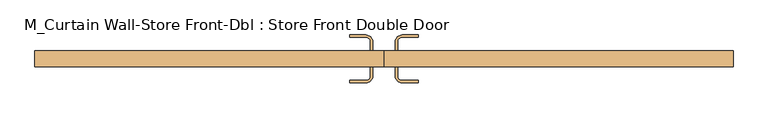
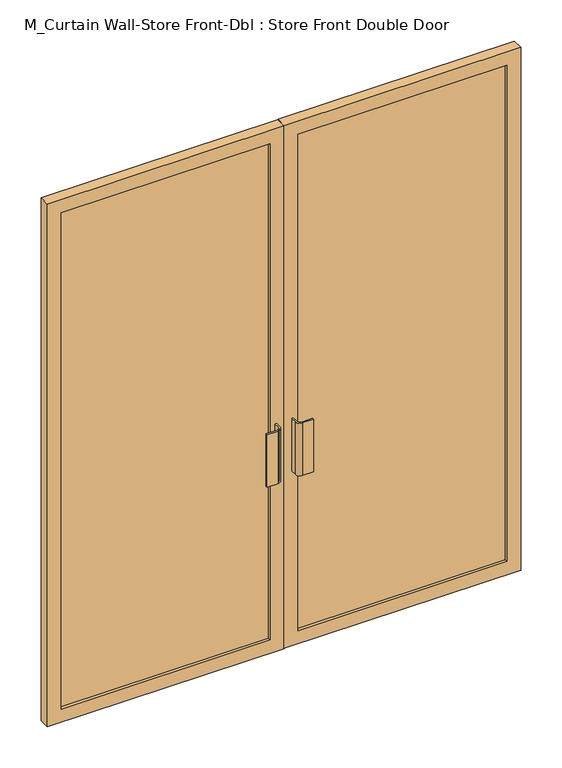
"""IFC4 building model written with IfcOpenShell, lengths in millimetres: door geometry, M_Curtain Wall-Store Front-Dbl : Store Front Double Door."""

from ifc_helpers import new_model, si_unit, point, frame, frame_2d, origin, place, context, project, spatial, polyline, circle_curve, trimmed, segment, composite_curve, outline, extrude, source, transform, mapped, element, save


def m_curtain_wall_store_front_dbl_store_front_double_door_7be21569(model_context):
    return source(origin(), model_context, "Body", "SweptSolid", [
        extrude(outline(composite_curve([segment(trimmed(circle_curve(frame_2d((-50.8, -14.85)), 19.05), [point((-31.75, -14.85))], [point((-50.8, -33.9))], False, "CARTESIAN"), True, "CONTINUOUS"), segment(polyline([(-50.8, -33.9), (-95.25, -33.9), (-95.25, -27.55), (-50.8, -27.55)]), True, "CONTINUOUS"), segment(trimmed(circle_curve(frame_2d((-50.8, -14.85)), 12.7), [point((-50.8, -27.55))], [point((-38.1, -14.85))], True, "CARTESIAN"), True, "CONTINUOUS"), segment(polyline([(-38.1, -14.85), (-38.1, 10.55), (-31.75, 10.55), (-31.75, -14.85)]), True, "CONTINUOUS")], self_intersect=False)), frame((0.0, 0.0, 762.0), z_axis=(0.0, 0.0, 1.0), x_axis=(1.0, 0.0, 0.0)), (0.0, 0.0, 1.0), 228.6),
        extrude(outline(composite_curve([segment(polyline([(31.75, -14.85), (31.75, 10.55), (38.1, 10.55), (38.1, -14.85)]), True, "CONTINUOUS"), segment(trimmed(circle_curve(frame_2d((50.8, -14.85)), 12.7), [point((38.1, -14.85))], [point((50.8, -27.55))], True, "CARTESIAN"), True, "CONTINUOUS"), segment(polyline([(50.8, -27.55), (95.25, -27.55), (95.25, -33.9), (50.8, -33.9)]), True, "CONTINUOUS"), segment(trimmed(circle_curve(frame_2d((50.8, -14.85)), 19.05), [point((50.8, -33.9))], [point((31.75, -14.85))], False, "CARTESIAN"), True, "CONTINUOUS")], self_intersect=False)), frame((0.0, 0.0, 762.0), z_axis=(0.0, 0.0, 1.0), x_axis=(1.0, 0.0, 0.0)), (0.0, 0.0, 1.0), 228.6),
        extrude(outline(composite_curve([segment(polyline([(-31.75, 80.4), (-31.75, 55.0), (-38.1, 55.0), (-38.1, 80.4)]), True, "CONTINUOUS"), segment(trimmed(circle_curve(frame_2d((-50.8, 80.4)), 12.7), [point((-38.1, 80.4))], [point((-50.8, 93.1))], True, "CARTESIAN"), True, "CONTINUOUS"), segment(polyline([(-50.8, 93.1), (-95.25, 93.1), (-95.25, 99.45), (-50.8, 99.45)]), True, "CONTINUOUS"), segment(trimmed(circle_curve(frame_2d((-50.8, 80.4)), 19.05), [point((-50.8, 99.45))], [point((-31.75, 80.4))], False, "CARTESIAN"), True, "CONTINUOUS")], self_intersect=False)), frame((0.0, 0.0, 762.0), z_axis=(0.0, 0.0, 1.0), x_axis=(1.0, 0.0, 0.0)), (0.0, 0.0, 1.0), 228.6),
        extrude(outline(composite_curve([segment(trimmed(circle_curve(frame_2d((50.8, 80.4)), 19.05), [point((31.75, 80.4))], [point((50.8, 99.45))], False, "CARTESIAN"), True, "CONTINUOUS"), segment(polyline([(50.8, 99.45), (95.25, 99.45), (95.25, 93.1), (50.8, 93.1)]), True, "CONTINUOUS"), segment(trimmed(circle_curve(frame_2d((50.8, 80.4)), 12.7), [point((50.8, 93.1))], [point((38.1, 80.4))], True, "CARTESIAN"), True, "CONTINUOUS"), segment(polyline([(38.1, 80.4), (38.1, 55.0), (31.75, 55.0), (31.75, 80.4)]), True, "CONTINUOUS")], self_intersect=False)), frame((0.0, 0.0, 762.0), z_axis=(0.0, 0.0, 1.0), x_axis=(1.0, 0.0, 0.0)), (0.0, 0.0, 1.0), 228.6),
        extrude(outline(polyline([(917.85, 23.25), (57.94375, 23.25), (57.94375, 42.3), (917.85, 42.3), (917.85, 23.25)])), frame((0.0, 0.0, 57.15), z_axis=(0.0, 0.0, 1.0), x_axis=(1.0, 0.0, 0.0)), (0.0, 0.0, 1.0), 2160.7),
        extrude(outline(polyline([(-57.94375, 23.25), (-917.85, 23.25), (-917.85, 42.3), (-57.94375, 42.3), (-57.94375, 23.25)])), frame((0.0, 0.0, 57.15), z_axis=(0.0, 0.0, 1.0), x_axis=(1.0, 0.0, 0.0)), (0.0, 0.0, 1.0), 2160.7),
        extrude(outline(polyline([(2275.0, 0.79375), (0.0, 0.79375), (0.0, 975.0), (2275.0, 975.0), (2275.0, 0.79375)]), holes=[polyline([(2217.85, 57.94375), (2217.85, 917.85), (57.15, 917.85), (57.15, 57.94375), (2217.85, 57.94375)])]), frame((0.0, 10.55, 0.0), z_axis=(0.0, 1.0, 0.0), x_axis=(0.0, 0.0, 1.0)), (0.0, 0.0, 1.0), 44.45),
        extrude(outline(polyline([(2275.0, -0.79375), (2275.0, -975.0), (0.0, -975.0), (0.0, -0.79375), (2275.0, -0.79375)]), holes=[polyline([(2217.85, -917.85), (2217.85, -57.94375), (57.15, -57.94375), (57.15, -917.85), (2217.85, -917.85)])]), frame((0.0, 10.55, 0.0), z_axis=(0.0, 1.0, 0.0), x_axis=(0.0, 0.0, 1.0)), (0.0, 0.0, 1.0), 44.45),
    ])


if __name__ == "__main__":
    model = new_model("IFC4")
    model_context = context("Model", 3, world=origin())
    ifc_project = project(units=[si_unit("LENGTHUNIT", "METRE", prefix="MILLI")], contexts=[model_context])
    site = spatial("IfcSite", under=ifc_project)
    building = spatial("IfcBuilding", under=site)
    placement = place(None, origin())
    m_curtain_wall_store_front_dbl_store_front_double_door_shape = m_curtain_wall_store_front_dbl_store_front_double_door_7be21569(model_context)
    element("IfcDoor", 1, ObjectType="M_Curtain Wall-Store Front-Dbl : Store Front Double Door", at=placement, inside=building, context=model_context, shape_type="MappedRepresentation", body=[
        mapped(m_curtain_wall_store_front_dbl_store_front_double_door_shape, transform((0.0, 0.0, 0.0), x_axis=(1.0, 0.0, 0.0), y_axis=(0.0, 1.0, 0.0), z_axis=(0.0, 0.0, 1.0))),
    ])
    save(model, "model.ifc")

# Revit data of these elements
# Type "M_Curtain Wall-Store Front-Dbl : Store Front Double Door"
#   Type Mark = "34"
#   Offset = 0.055 m
#   Function = 1
#   Define Thermal Properties by = 1
#   Material = Metal - Aluminum
#   Glazing Material = Window - Glass
#   Assembly Code = ""
# Element 1 (IfcDoor, "M_Curtain Wall-Store Front-Dbl : Store Front Double Door")
#   Materials on its faces: "Metal - Aluminum", "Window - Glass"
# Materials
#   "Metal - Aluminum": class "Unassigned", colour RGB 247 247 247, transparency 0, Comments = "Rendering appearance not upgraded "
#   "Window - Glass": class "Glas", colour RGB 128 128 255, transparency 0.75
